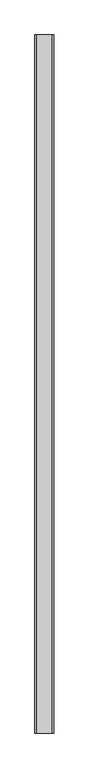
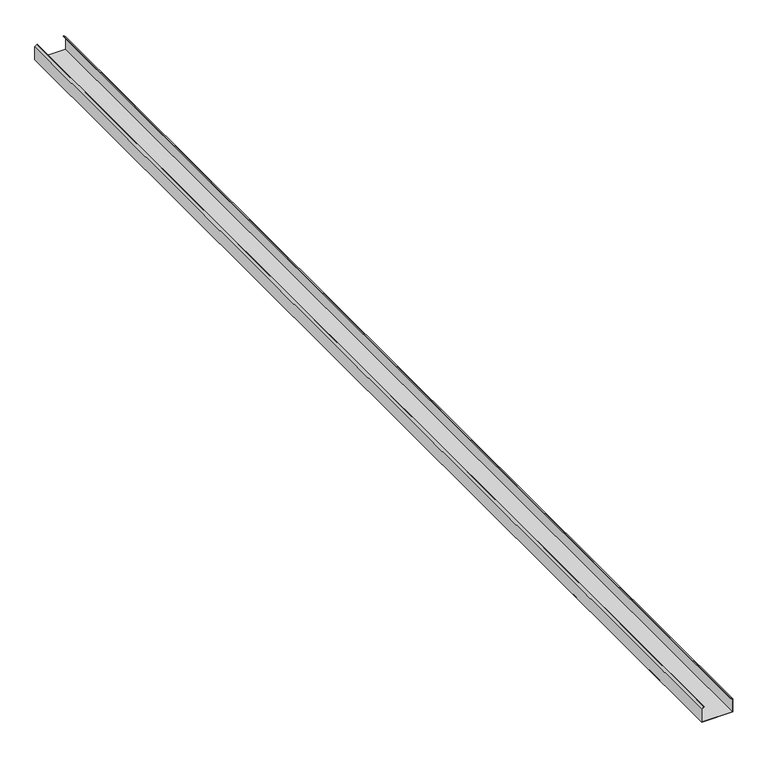
"""IFC4 building model written with IfcOpenShell, lengths in millimetres: proxy geometry, Generic Models 7:Generic Models 1:1:Generic Models 1:1 : Generic Models 7:Generic Models 1:337419:31 : Generic Models 7:Generic Models 1:1:Generic Models 1:1 : Generic Models 7:Generic Models 1:337419:306201."""

from ifc_helpers import new_model, si_unit, frame, origin, place, context, project, spatial, polyline, outline, extrude, source, transform, mapped, element, save


def generic_models_6bacda05(model_context):
    return source(origin(), model_context, "Body", "SweptSolid", [
        extrude(outline(polyline([(3617.9125, 667293.3117239), (3617.9125, 667496.5117239), (3706.8125, 667496.5117239), (3719.057604, 667481.9185773), (3716.9294367, 667480.132833), (3705.517039, 667493.7335989), (3620.690625, 667493.7335989), (3620.690625, 667296.0898489), (3705.517039, 667296.0898489), (3716.9294367, 667309.6906149), (3719.057604, 667307.9048706), (3706.8125, 667293.3117239), (3617.9125, 667293.3117239)])), frame((0.0, -507687.0163841, 0.0), z_axis=(0.0, 1.0, 0.0), x_axis=(0.0, 0.0, 1.0)), (0.0, 0.0, 1.0), 7569.2),
    ])


if __name__ == "__main__":
    model = new_model("IFC4")
    model_context = context("Model", 3, world=origin())
    ifc_project = project(units=[si_unit("LENGTHUNIT", "METRE", prefix="MILLI")], contexts=[model_context])
    site = spatial("IfcSite", under=ifc_project)
    building = spatial("IfcBuilding", under=site)
    placement = place(None, origin())
    generic_models_shape = generic_models_6bacda05(model_context)
    element("IfcBuildingElementProxy", 1, Name="Generic Models 7:Generic Models 1:1:Generic Models 1:1 : Generic Models 7:Generic Models 1:337419:31 : Generic Models 7:Generic Models 1:1:Generic Models 1:1 : Generic Models 7:Generic Models 1:337419:306201", ObjectType="Generic Models 7:Generic Models 1:1:Generic Models 1:1 : Generic Models 7:Generic Models 1:337419:31 : Generic Models 7:Generic Models 1:1:Generic Models 1:1 : Generic Models 7:Generic Models 1:337419:306201", at=placement, inside=building, context=model_context, shape_type="MappedRepresentation", body=[
        mapped(generic_models_shape, transform((0.0, 0.0, 0.0), x_axis=(1.0, 0.0, 0.0), y_axis=(0.0, 1.0, 0.0), z_axis=(0.0, 0.0, 1.0))),
    ])
    save(model, "model.ifc")

# Revit data of these elements
# Type "Generic Models 7:Generic Models 1:1:Generic Models 1:1 : Generic Models 7:Generic Models 1:337419:31 : Generic Models 7:Generic Models 1:1:Generic Models 1:1 : Generic Models 7:Generic Models 1:337419:306201"
#   NameOverride = "Generic Models 7:Generic Models 1:1:Generic Models 1:1 : Generic Models 7:Generic Models 1:337419:306201"
#   ObjectTypeOverride = "Generic Models 1:1 : Generic Models 7:Generic Models 1:337419"
#   Reference = "Generic Models 1"
#   Tag = "306201"
# Element 1 (IfcBuildingElementProxy, "Generic Models 7:Generic Models 1:1:Generic Models 1:1 : Generic Models 7:Generic Models 1:337419:31 : Generic Models 7:Generic Models 1:1:Generic Models 1:1 : Generic Models 7:Generic Models 1:337419:306201")
#   Materials on its faces: "CEE' SECTION (8.0x3.5C - SEE STRUCT. DWGS)"
# Materials
#   "CEE' SECTION (8.0x3.5C - SEE STRUCT. DWGS)": class "Unassigned", colour RGB 210 209 208, transparency 0, Keynote = "M05121300.02", Cost = 0
